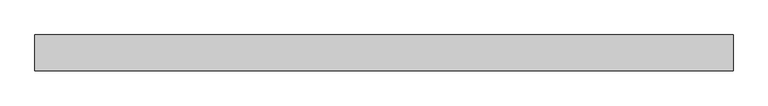
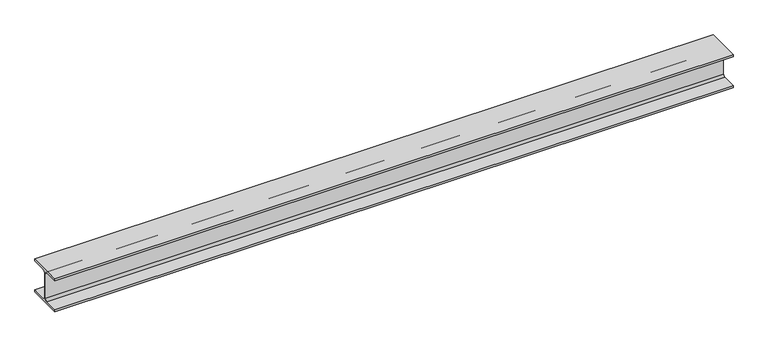
"""IFC4 building model written with IfcOpenShell, lengths in millimetres: beam geometry, 0912_Steel Framing_H-KSD3502 : H_SB_ASB_H-200x200x8x12."""

from ifc_helpers import new_model, si_unit, point, frame, frame_2d, origin, place, context, project, spatial, polyline, circle_curve, trimmed, segment, composite_curve, outline, extrude, source, transform, mapped, element, save


def beam_cfb84a49(model_context):
    return source(origin(), model_context, "Body", "SweptSolid", [
        extrude(outline(composite_curve([segment(polyline([(100.0, -88.0), (100.0, -100.0), (-100.0, -100.0), (-100.0, -88.0), (-17.0, -88.0)]), True, "CONTINUOUS"), segment(trimmed(circle_curve(frame_2d((-17.0, -75.0)), 13.0), [point((-17.0, -88.0))], [point((-4.0, -75.0))], True, "CARTESIAN"), True, "CONTINUOUS"), segment(polyline([(-4.0, -75.0), (-4.0, 75.0)]), True, "CONTINUOUS"), segment(trimmed(circle_curve(frame_2d((-17.0, 75.0)), 13.0), [point((-4.0, 75.0))], [point((-17.0, 88.0))], True, "CARTESIAN"), True, "CONTINUOUS"), segment(polyline([(-17.0, 88.0), (-100.0, 88.0), (-100.0, 100.0), (100.0, 100.0), (100.0, 88.0), (17.0, 88.0)]), True, "CONTINUOUS"), segment(trimmed(circle_curve(frame_2d((17.0, 75.0)), 13.0), [point((17.0, 88.0))], [point((4.0, 75.0))], True, "CARTESIAN"), True, "CONTINUOUS"), segment(polyline([(4.0, 75.0), (4.0, -75.0)]), True, "CONTINUOUS"), segment(trimmed(circle_curve(frame_2d((17.0, -75.0)), 13.0), [point((4.0, -75.0))], [point((17.0, -88.0))], True, "CARTESIAN"), True, "CONTINUOUS"), segment(polyline([(17.0, -88.0), (100.0, -88.0)]), True, "CONTINUOUS")], self_intersect=False)), frame((-1909.0326226, 0.0, 0.0), z_axis=(1.0, 0.0, 0.0), x_axis=(0.0, 1.0, 0.0)), (0.0, 0.0, 1.0), 3902.9065136),
    ])


if __name__ == "__main__":
    model = new_model("IFC4")
    model_context = context("Model", 3, world=origin())
    ifc_project = project(units=[si_unit("LENGTHUNIT", "METRE", prefix="MILLI")], contexts=[model_context])
    site = spatial("IfcSite", under=ifc_project)
    building = spatial("IfcBuilding", under=site)
    placement = place(None, origin())
    beam_shape = beam_cfb84a49(model_context)
    element("IfcBeam", 1, ObjectType="0912_Steel Framing_H-KSD3502 : H_SB_ASB_H-200x200x8x12", at=placement, inside=building, context=model_context, shape_type="MappedRepresentation", body=[
        mapped(beam_shape, transform((0.0, 0.0, 0.0), x_axis=(1.0, 0.0, 0.0), y_axis=(0.0, 1.0, 0.0), z_axis=(0.0, 0.0, 1.0))),
    ])
    save(model, "model.ifc")

# Revit data of these elements
# Type "0912_Steel Framing_H-KSD3502 : H_SB_ASB_H-200x200x8x12"
#   H_WM Code_1 = "S01AA002-00001 | Main Steel Structure Fabrication Work | Shelter/Building | Medium Steel - Standard (90KG/M>Weight≥30KG/M) | Material: (   )"
#   H_WM Code_2 = "S03AA028-00001 | Main Steel Structure Erection Work | Shelter/Building | Medium Steel (90KG/M>Weight≥30KG/M) | Material: (   )"
#   H_WM Code_3 = "S01AA010-00001 | Main Steel Structure Fabrication Work | Shelter/Building | Steel Painting/Coating | for Non-Fireproofed Steel Surface, Surface Preparation, Primer, Second & Final Coat | Material: (   )"
#   H_Q'ty Cal Type Tag = "SB-Q2"
#   Width = 20.0 cm
#   Web Thickness = 0.8 cm
#   Web Fillet = 1.3 cm
#   Warping Constant = 141000.0 cm⁶
#   W = 0
#   Torsional Moment of Inertia = 26.2485 cm⁴
#   Section Area = 63.53 cm²
#   Plastic Modulus weak axis = 244.0 cm³
#   Plastic Modulus strong axis = 525.0 cm³
#   Perimeter = 1.16 m²/m
#   Nominal Weight = 49.90 kgf/m
#   Moment of Inertia weak axis = 1600.00 cm⁴
#   Moment of Inertia strong axis = 4720.00 cm⁴
#   Height = 20.0 cm
#   Flange Thickness = 1.2 cm
#   Elastic Modulus weak axis = 160.0 cm³
#   Elastic Modulus strong axis = 472.0 cm³
#   Centroid Vertical = 10.0 cm
#   Centroid Horizontal = 10.0 cm
#   Ix = 47200000
#   Length [instance default] = 1.5240 m
#   Zx = 525000
#   b = 0.2000 m
#   h = 0.2000 m
#   r = 0.0130 m
#   s = 0.0080 m
#   t = 0.0120 m
#   A = 0.006353 m²
#   Structural Material [instance default] = Steel, 45-345
#   Assembly Code = ""
# Element 1 (IfcBeam, "0912_Steel Framing_H-KSD3502 : H_SB_ASB_H-200x200x8x12")
#   Structural Material = none
# Materials
#   "Steel, 45-345": class "Metal", colour RGB 189 187 185, transparency 0, Description = "Steel 345 MPa", Cost = 0
